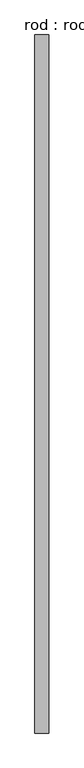
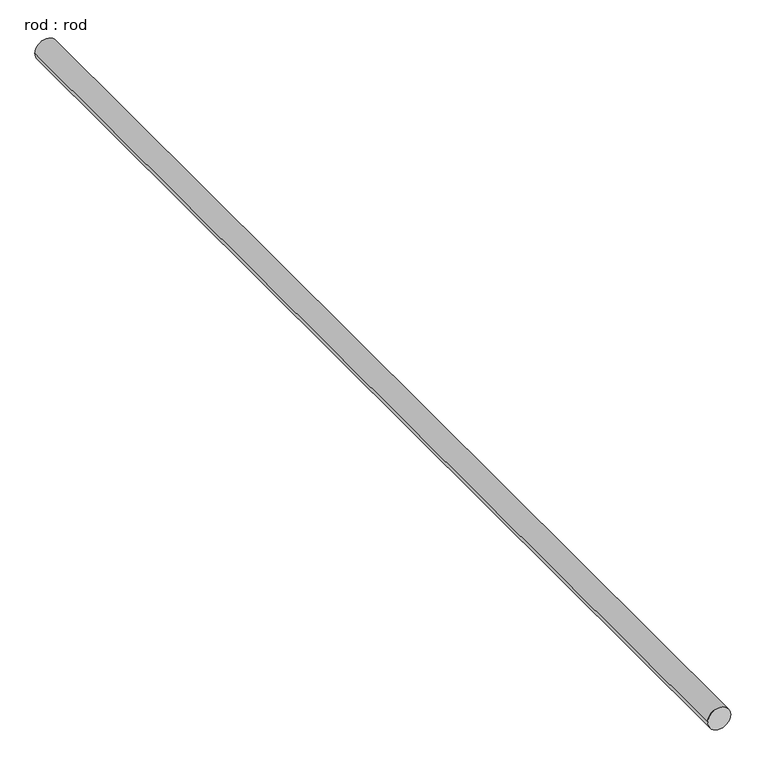
"""IFC4 building model written with IfcOpenShell, lengths in millimetres: proxy geometry, rod : rod."""

from ifc_helpers import new_model, si_unit, point, frame, frame_2d, origin, place, context, project, spatial, circle_curve, trimmed, segment, composite_curve, outline, extrude, source, transform, mapped, element, save


def rod_rod_32803c68(model_context):
    return source(origin(), model_context, "Body", "SweptSolid", [
        extrude(outline(composite_curve([segment(trimmed(circle_curve(frame_2d((0.0108462, 0.0)), 200.0), [point((0.0108462, 200.0))], [point((0.0108462, -200.0))], False, "CARTESIAN"), True, "CONTINUOUS"), segment(trimmed(circle_curve(frame_2d((0.0108462, 0.0)), 200.0), [point((0.0108462, -200.0))], [point((0.0108462, 200.0))], False, "CARTESIAN"), True, "CONTINUOUS")], self_intersect=False)), frame((0.0, -6066.1029891, 0.0), z_axis=(0.0, 1.0, 0.0), x_axis=(0.0, 0.0, 1.0)), (0.0, 0.0, 1.0), 20317.6632089),
    ])


if __name__ == "__main__":
    model = new_model("IFC4")
    model_context = context("Model", 3, world=origin())
    ifc_project = project(units=[si_unit("LENGTHUNIT", "METRE", prefix="MILLI")], contexts=[model_context])
    site = spatial("IfcSite", under=ifc_project)
    building = spatial("IfcBuilding", under=site)
    placement = place(None, origin())
    rod_rod_shape = rod_rod_32803c68(model_context)
    element("IfcBuildingElementProxy", 1, Name="rod : rod", ObjectType="rod : rod", at=placement, inside=building, context=model_context, shape_type="MappedRepresentation", body=[
        mapped(rod_rod_shape, transform((0.0, 0.0, 0.0), x_axis=(1.0, 0.0, 0.0), y_axis=(0.0, 1.0, 0.0), z_axis=(0.0, 0.0, 1.0))),
    ])
    save(model, "model.ifc")

# Revit data of these elements
# Type "rod : rod"
#   Default Elevation = 0
